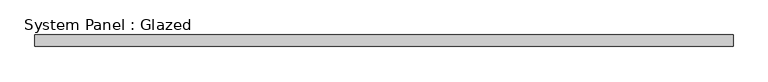
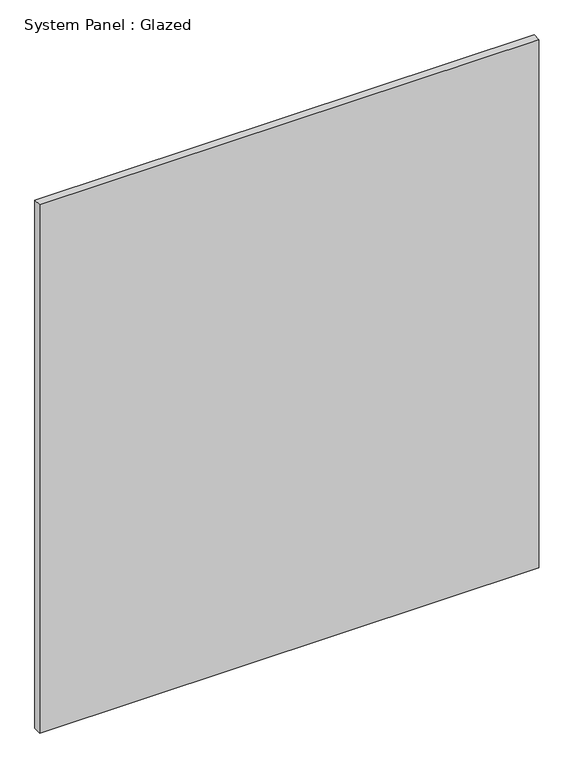
"""IFC4 building model written with IfcOpenShell, lengths in millimetres: plate geometry, System Panel : Glazed."""

from ifc_helpers import new_model, si_unit, origin, origin_with_axes, place, context, project, spatial, polyline, outline, extrude, source, transform, mapped, element, save


def system_panel_glazed_11080212(model_context):
    return source(origin(), model_context, "Body", "SweptSolid", [
        extrude(outline(polyline([(755.5084626, 24.5), (-755.5084626, 24.5), (-755.5084626, 49.5), (755.5084626, 49.5), (755.5084626, 24.5)])), origin_with_axes(), (0.0, 0.0, 1.0), 1690.2939092),
    ])


if __name__ == "__main__":
    model = new_model("IFC4")
    model_context = context("Model", 3, world=origin())
    ifc_project = project(units=[si_unit("LENGTHUNIT", "METRE", prefix="MILLI")], contexts=[model_context])
    site = spatial("IfcSite", under=ifc_project)
    building = spatial("IfcBuilding", under=site)
    placement = place(None, origin())
    system_panel_glazed_shape = system_panel_glazed_11080212(model_context)
    element("IfcPlate", 1, ObjectType="System Panel : Glazed", at=placement, inside=building, context=model_context, shape_type="MappedRepresentation", body=[
        mapped(system_panel_glazed_shape, transform((0.0, 0.0, 0.0), x_axis=(1.0, 0.0, 0.0), y_axis=(0.0, 1.0, 0.0), z_axis=(0.0, 0.0, 1.0))),
    ])
    save(model, "model.ifc")

# Revit data of these elements
# Element 1 (IfcPlate, "System Panel : Glazed")
#   Materials on its faces: "Glass"
# Materials
#   "Glass": class "Glass", colour RGB 218 227 224, transparency 0.85, Description = "Soda Lime Glass", Cost = 0
